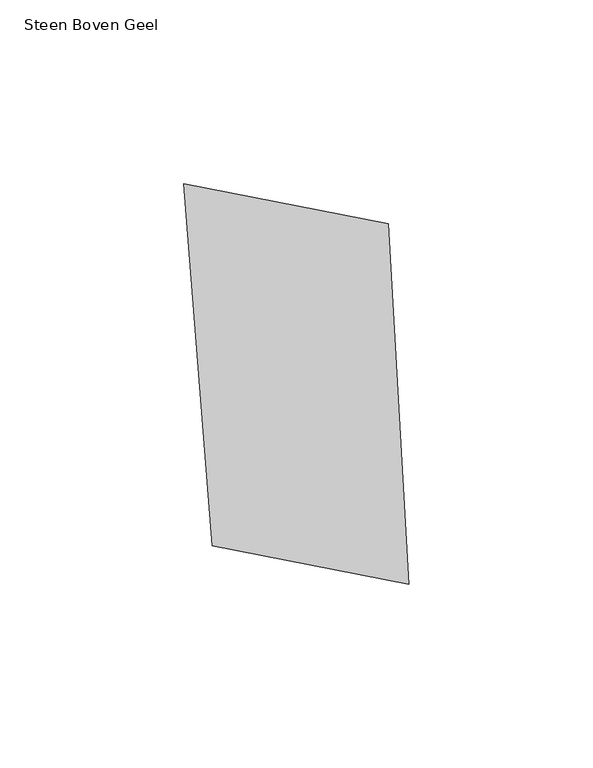
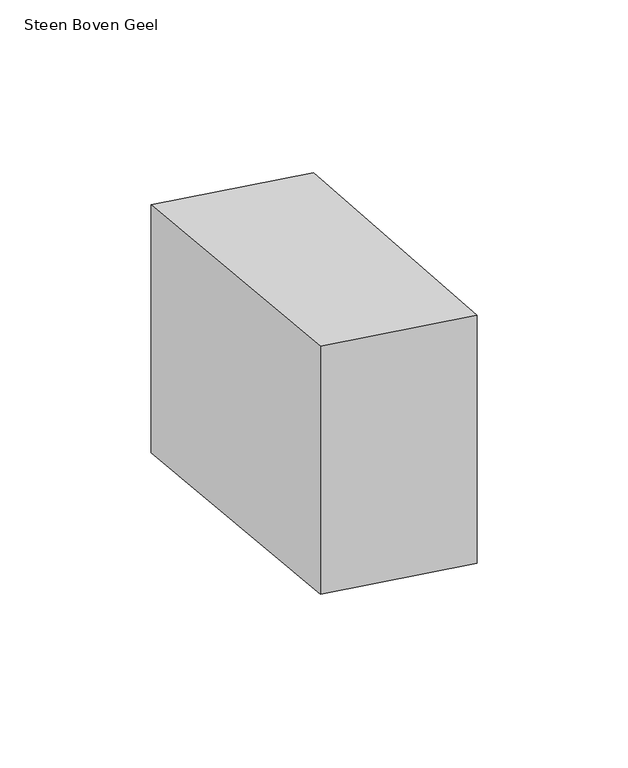
"""IFC4 building model written with IfcOpenShell, lengths in millimetres: proxy geometry, 00_GMA_steen_versie_4 : Steen Boven Geel."""

from ifc_helpers import new_model, si_unit, origin, origin_with_axes, place, context, project, spatial, polyline, outline, extrude, source, transform, mapped, element, save


def steen_boven_geel_6a5d1924(model_context):
    return source(origin(), model_context, "Body", "SweptSolid", [
        extrude(outline(polyline([(97.6808907, 121.0756012), (103.3228543, 23.0219895), (49.7836371, 33.446677), (42.0632898, 131.9288766), (97.6808907, 121.0756012)])), origin_with_axes(), (0.0, 0.0, 1.0), 100.0),
    ])


if __name__ == "__main__":
    model = new_model("IFC4")
    model_context = context("Model", 3, world=origin())
    ifc_project = project(units=[si_unit("LENGTHUNIT", "METRE", prefix="MILLI")], contexts=[model_context])
    site = spatial("IfcSite", under=ifc_project)
    building = spatial("IfcBuilding", under=site)
    placement = place(None, origin())
    steen_boven_geel_shape = steen_boven_geel_6a5d1924(model_context)
    element("IfcBuildingElementProxy", 1, Name="00_GMA_steen_versie_4 : Steen Boven Geel", ObjectType="00_GMA_steen_versie_4 : Steen Boven Geel", at=placement, inside=building, context=model_context, shape_type="MappedRepresentation", body=[
        mapped(steen_boven_geel_shape, transform((0.0, 0.0, 0.0), x_axis=(1.0, 0.0, 0.0), y_axis=(0.0, 1.0, 0.0), z_axis=(0.0, 0.0, 1.0))),
    ])
    save(model, "model.ifc")

# Revit data of these elements
# Type "00_GMA_steen_versie_4 : Steen Boven Geel"
#   StootVoegHalfBoven [instance default] = 5 mm
#   StootVoegHalf [instance default] = 5 mm
#   StootVoegBreedteOnder = 10 mm
#   StootVoegBreedteBoven = 10 mm
#   Steendikte = 100 mm
#   LintVoegOnderHalf = 5 mm
#   LintVoegOnder = 10 mm
#   LintVoegBovenHalf = 0 mm
#   LintVoegBoven = 0 mm
#   materiaal = 21_steen_geel
#   MateriaalVoeg = none
#   Default Elevation = 0
# Element 1 (IfcBuildingElementProxy, "00_GMA_steen_versie_4 : Steen Boven Geel")
#   Materials on its faces: "21_steen_geel"
# Materials
#   "21_steen_geel": class "Unassigned", colour RGB 202 202 0, transparency 0, Cost = 0
